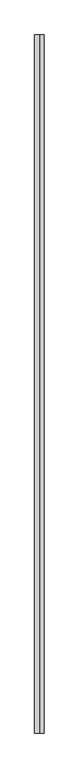
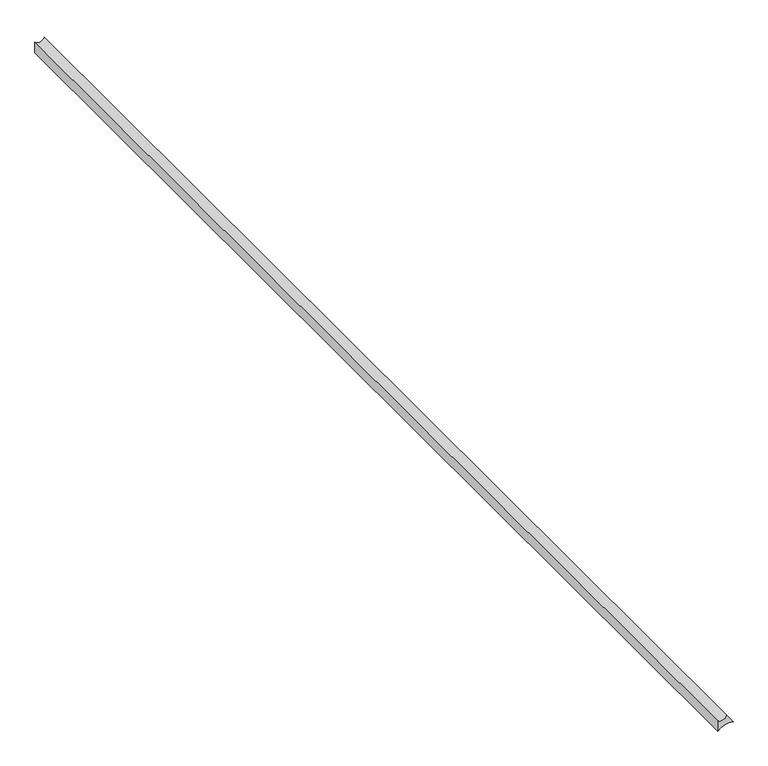
"""IFC4 building model written with IfcOpenShell, lengths in millimetres: proxy geometry, Joint045 17386 : Joint045 17386."""

from ifc_helpers import new_model, si_unit, point, frame, frame_2d, origin, place, context, project, spatial, polyline, circle_curve, trimmed, segment, composite_curve, outline, extrude, source, transform, mapped, element, save


def generic_models_7c192336(model_context):
    return source(origin(), model_context, "Body", "SweptSolid", [
        extrude(outline(composite_curve([segment(polyline([(41324.6855963, 6175.6039248), (41340.0941189, 6164.6952008)]), True, "CONTINUOUS"), segment(trimmed(circle_curve(frame_2d((41342.4096103, 6155.7718668)), 9.2188606), [point((41340.0941189, 6164.6952008))], [point((41335.9078778, 6149.2362057))], True, "CARTESIAN"), True, "CONTINUOUS"), segment(polyline([(41335.9078778, 6149.2362057), (41317.0542113, 6149.2362057)]), True, "CONTINUOUS"), segment(trimmed(circle_curve(frame_2d((41290.4573004, 6171.2221267)), 34.507628), [point((41317.0542113, 6149.2362057))], [point((41324.6855963, 6175.6039248))], True, "CARTESIAN"), True, "CONTINUOUS")], self_intersect=False)), frame((0.0, 2217.3609988, 0.0), z_axis=(0.0, 1.0, 0.0), x_axis=(0.0, 0.0, 1.0)), (0.0, 0.0, 1.0), 2000.0),
    ])


if __name__ == "__main__":
    model = new_model("IFC4")
    model_context = context("Model", 3, world=origin())
    ifc_project = project(units=[si_unit("LENGTHUNIT", "METRE", prefix="MILLI")], contexts=[model_context])
    site = spatial("IfcSite", under=ifc_project)
    building = spatial("IfcBuilding", under=site)
    placement = place(None, origin())
    generic_models_shape = generic_models_7c192336(model_context)
    element("IfcBuildingElementProxy", 1, Name="Joint045 17386 : Joint045 17386", ObjectType="Joint045 17386 : Joint045 17386", at=placement, inside=building, context=model_context, shape_type="MappedRepresentation", body=[
        mapped(generic_models_shape, transform((0.0, 0.0, 0.0), x_axis=(1.0, 0.0, 0.0), y_axis=(0.0, 1.0, 0.0), z_axis=(0.0, 0.0, 1.0))),
    ])
    save(model, "model.ifc")

# Revit data of these elements
# Type "Joint045 17386 : Joint045 17386"
#   NameOverride = "Joint045"
# Element 1 (IfcBuildingElementProxy, "Joint045 17386 : Joint045 17386")
#   Materials on its faces: "SEALANT"
# Materials
#   "SEALANT": class "Unassigned", colour RGB 142 225 148, transparency 0
